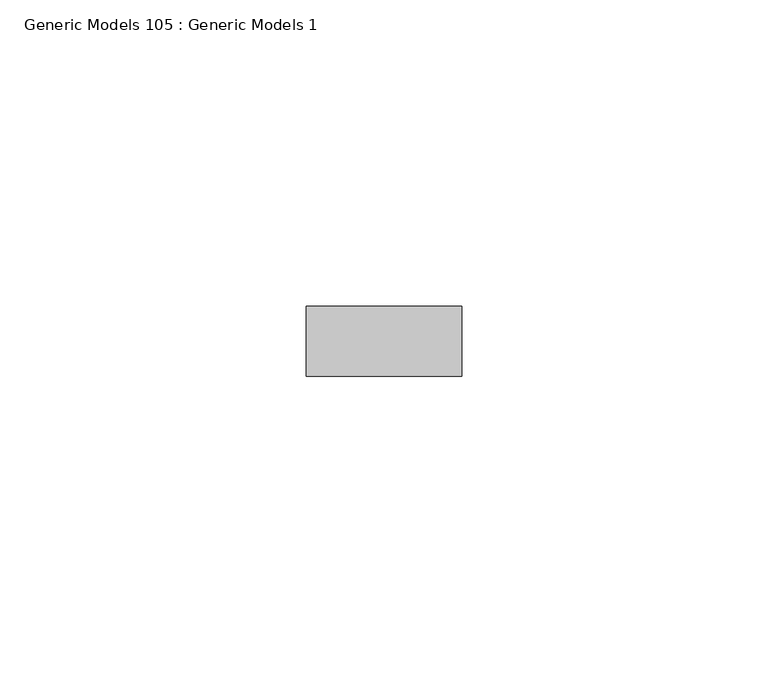
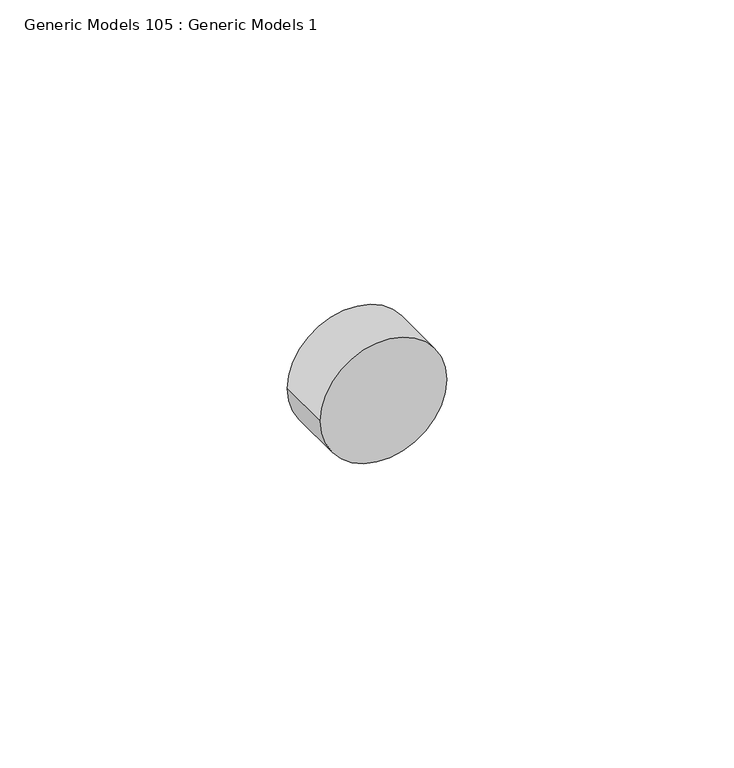
"""IFC4 building model written with IfcOpenShell, lengths in millimetres: proxy geometry, Generic Models 105 : Generic Models 1."""

import ifcopenshell
import ifcopenshell.guid

model = None  # the IFC model being written
_history = None  # IfcOwnerHistory: only IFC2X3 demands one
_inside = {}  # id of a spatial element -> (the spatial element, [elements in it])
_under = {}  # id of a project, library or spatial element -> (it, [spatial elements below it])
_declared = {}  # id of a project -> (the project, [libraries it declares])
_typed = {}  # id of a type object -> (the type object, [elements of that type])
_made_of = {}  # id of a material, layer set ... -> (it, [elements and type objects made of it])


def new_model(schema):
    """Start an empty IFC model of exactly this schema.

    Asked for "IFC4X3", IfcOpenShell would pick the latest addendum, in which some entities
    have other attributes; the version numbers below select the first issue.
    IFC2X3 requires an IfcOwnerHistory on every rooted entity: one is made here for all.
    """
    global model, _history
    if schema == "IFC4X3":
        model = ifcopenshell.file(schema_version=(4, 3, 0, 0))
    else:
        model = ifcopenshell.file(schema=schema)
    _inside.clear()
    _under.clear()
    _declared.clear()
    _typed.clear()
    _made_of.clear()
    _history = None
    if model.schema == "IFC2X3":
        org = make("IfcOrganization", Name="unknown")
        user = make(
            "IfcPersonAndOrganization",
            ThePerson=make("IfcPerson", FamilyName="unknown"),
            TheOrganization=org,
        )
        app = make(
            "IfcApplication",
            ApplicationDeveloper=org,
            Version="unknown",
            ApplicationFullName="unknown",
            ApplicationIdentifier="unknown",
        )
        _history = make(
            "IfcOwnerHistory",
            OwningUser=user,
            OwningApplication=app,
            ChangeAction="ADDED",
            CreationDate=0,
        )
    return model


def make(cls, **values):
    """One entity of the class cls with the attributes given. An attribute that is None is left unset."""
    return model.create_entity(
        cls, **{name: value for name, value in values.items() if value is not None}
    )


def rooted(cls, **values):
    """An entity with a GlobalId (a new one), such as an element, a storey or a relation."""
    return make(cls, GlobalId=ifcopenshell.guid.new(), OwnerHistory=_history, **values)


def si_unit(unit_type, name, prefix=None):
    """IfcSIUnit, for example si_unit("LENGTHUNIT", "METRE", prefix="MILLI")."""
    return make("IfcSIUnit", UnitType=unit_type, Prefix=prefix, Name=name)


def assignment(units):
    """IfcUnitAssignment: the units of a project."""
    return None if units is None else make("IfcUnitAssignment", Units=units)


def point(xyz):
    """IfcCartesianPoint."""
    return None if xyz is None else make("IfcCartesianPoint", Coordinates=xyz)


def direction(xyz):
    """IfcDirection."""
    return None if xyz is None else make("IfcDirection", DirectionRatios=xyz)


def frame(location, z_axis=None, x_axis=None):
    """IfcAxis2Placement3D, a coordinate frame: its origin and axes. An axis left out is left unset."""
    return make(
        "IfcAxis2Placement3D",
        Location=point(location),
        Axis=direction(z_axis),
        RefDirection=direction(x_axis),
    )


def frame_2d(location, x_axis=None):
    """IfcAxis2Placement2D, a coordinate frame in the plane: its origin and x axis."""
    return make(
        "IfcAxis2Placement2D", Location=point(location), RefDirection=direction(x_axis)
    )


def origin():
    """The frame at (0, 0, 0) with its axes left unset."""
    return frame((0.0, 0.0, 0.0))


def place(relative_to, where):
    """IfcLocalPlacement: puts the frame where relative to a parent placement (None: the world)."""
    return make(
        "IfcLocalPlacement", PlacementRelTo=relative_to, RelativePlacement=where
    )


def context(
    kind, dimensions, precision=None, world=None, true_north=None, identifier=None
):
    """IfcGeometricRepresentationContext, for example the 3D "Model" context."""
    return make(
        "IfcGeometricRepresentationContext",
        ContextIdentifier=identifier,
        ContextType=kind,
        CoordinateSpaceDimension=dimensions,
        Precision=precision,
        WorldCoordinateSystem=world,
        TrueNorth=true_north,
    )


def project(units=None, contexts=None):
    """IfcProject with its units and contexts."""
    return rooted(
        "IfcProject",
        Name="project",
        RepresentationContexts=contexts,
        UnitsInContext=assignment(units),
    )


def spatial(cls, under=None, at=None, **own):
    """A site, building, storey or space (cls), placed at a placement, below another one or the project."""
    s = rooted(cls, ObjectPlacement=at, **own)
    if under is not None:
        _under.setdefault(under.id(), (under, []))[1].append(s)
    return s


def circle_curve(where, radius):
    """IfcCircle in the frame where."""
    return make("IfcCircle", Position=where, Radius=radius)


def trimmed(basis, trim1, trim2, sense, master):
    """IfcTrimmedCurve: the piece of a basis curve between two trims."""
    return make(
        "IfcTrimmedCurve",
        BasisCurve=basis,
        Trim1=trim1,
        Trim2=trim2,
        SenseAgreement=sense,
        MasterRepresentation=master,
    )


def segment(curve, same_sense, transition):
    """IfcCompositeCurveSegment."""
    return make(
        "IfcCompositeCurveSegment",
        Transition=transition,
        SameSense=same_sense,
        ParentCurve=curve,
    )


def composite_curve(segments, self_intersect=None):
    """IfcCompositeCurve: segments joined end to end."""
    return make("IfcCompositeCurve", Segments=segments, SelfIntersect=self_intersect)


def outline(outer, holes=None, kind="AREA"):
    """IfcArbitraryClosedProfileDef: a profile drawn as a closed curve; with holes, ...WithVoids."""
    if holes is None:
        return make("IfcArbitraryClosedProfileDef", ProfileType=kind, OuterCurve=outer)
    return make(
        "IfcArbitraryProfileDefWithVoids",
        ProfileType=kind,
        OuterCurve=outer,
        InnerCurves=holes,
    )


def extrude(swept, where, along, depth):
    """IfcExtrudedAreaSolid: the profile swept, set in the frame where, extruded along a direction by depth."""
    return make(
        "IfcExtrudedAreaSolid",
        SweptArea=swept,
        Position=where,
        ExtrudedDirection=direction(along),
        Depth=depth,
    )


def shape(context_of_items, identifier, shape_type, items):
    """IfcShapeRepresentation: the items that make up one representation, for example the "Body"."""
    return make(
        "IfcShapeRepresentation",
        ContextOfItems=context_of_items,
        RepresentationIdentifier=identifier,
        RepresentationType=shape_type,
        Items=items,
    )


def source(mapping_origin, context_of_items, identifier, shape_type, items):
    """IfcRepresentationMap: a shape defined once, which mapped items show again and again."""
    return make(
        "IfcRepresentationMap",
        MappingOrigin=mapping_origin,
        MappedRepresentation=shape(context_of_items, identifier, shape_type, items),
    )


def transform(
    local_origin,
    x_axis=None,
    y_axis=None,
    z_axis=None,
    scale=None,
    scale2=None,
    scale3=None,
    uniform=True,
):
    """IfcCartesianTransformationOperator3D, or its non-uniform kind. x_axis, y_axis, z_axis: its Axis1, 2, 3."""
    if uniform:
        return make(
            "IfcCartesianTransformationOperator3D",
            Axis1=direction(x_axis),
            Axis2=direction(y_axis),
            LocalOrigin=point(local_origin),
            Scale=scale,
            Axis3=direction(z_axis),
        )
    return make(
        "IfcCartesianTransformationOperator3DnonUniform",
        Axis1=direction(x_axis),
        Axis2=direction(y_axis),
        LocalOrigin=point(local_origin),
        Scale=scale,
        Axis3=direction(z_axis),
        Scale2=scale2,
        Scale3=scale3,
    )


def mapped(mapping_source, mapping_target):
    """IfcMappedItem: shows the shape of a source again, moved by a transform."""
    return make(
        "IfcMappedItem", MappingSource=mapping_source, MappingTarget=mapping_target
    )


def made_of(thing, what):
    """Note that an element or type object is made of a material, layer set ...; save() writes the relation."""
    if what is not None:
        _made_of.setdefault(what.id(), (what, []))[1].append(thing)
    return thing


def element(
    cls,
    number,
    at=None,
    inside=None,
    cuts=None,
    type_object=None,
    material=None,
    context=None,
    identifier="Body",
    shape_type=None,
    held_by="IfcProductDefinitionShape",
    body=None,
    shapes=None,
    **own,
):
    """One element of the class cls, such as IfcWall. Its Tag is "e" and its number.

    at: its placement. inside: the storey or other place that contains it. cuts: it is an
    opening in that element (IfcRelVoidsElement). A single representation is given by context,
    identifier, shape_type and body (its items); several are given by shapes. held_by: the class
    of the entity that holds the representations. save() writes the other relations.
    """
    e = rooted(cls, Tag="e%d" % number, ObjectPlacement=at, **own)
    if body is not None:
        shapes = [shape(context, identifier, shape_type, body)]
    if shapes is not None:
        e.Representation = make(held_by, Representations=shapes)
    if inside is not None:
        _inside.setdefault(inside.id(), (inside, []))[1].append(e)
    if cuts is not None:
        rooted(
            "IfcRelVoidsElement", RelatingBuildingElement=cuts, RelatedOpeningElement=e
        )
    if type_object is not None:
        _typed.setdefault(type_object.id(), (type_object, []))[1].append(e)
    return made_of(e, material)


def aggregate(whole, parts):
    """IfcRelAggregates: a whole, such as a stair, and the parts it consists of."""
    return rooted("IfcRelAggregates", RelatingObject=whole, RelatedObjects=parts)


def save(model, path):
    """Write the relations noted so far, then the file.

    IfcRelAggregates (storeys below a building ...), IfcRelContainedInSpatialStructure (elements
    in a storey), IfcRelDefinesByType, IfcRelAssociatesMaterial and IfcRelDeclares: one each for
    every whole, place, type object, material and project.
    """
    for whole, parts in _under.values():
        aggregate(whole, parts)
    for where, things in _inside.values():
        rooted(
            "IfcRelContainedInSpatialStructure",
            RelatedElements=things,
            RelatingStructure=where,
        )
    for kind, things in _typed.values():
        rooted("IfcRelDefinesByType", RelatedObjects=things, RelatingType=kind)
    for what, things in _made_of.values():
        rooted("IfcRelAssociatesMaterial", RelatedObjects=things, RelatingMaterial=what)
    for by, libraries in _declared.values():
        rooted("IfcRelDeclares", RelatingContext=by, RelatedDefinitions=libraries)
    model.write(path)


def generic_models_105_generic_models_1_8c8b2fa9(model_context):
    return source(origin(), model_context, "Body", "SweptSolid", [
        extrude(outline(composite_curve([segment(trimmed(circle_curve(frame_2d((37517.3905034, 6289.9828124)), 12.7), [point((37517.3905034, 6277.2828124))], [point((37517.3905034, 6302.6828124))], False, "CARTESIAN"), True, "CONTINUOUS"), segment(trimmed(circle_curve(frame_2d((37517.3905034, 6289.9828124)), 12.7), [point((37517.3905034, 6302.6828124))], [point((37517.3905034, 6277.2828124))], False, "CARTESIAN"), True, "CONTINUOUS")], self_intersect=False)), frame((0.0, 1836.9202358, 0.0), z_axis=(0.0, 1.0, 0.0), x_axis=(0.0, 0.0, 1.0)), (0.0, 0.0, 1.0), 11.4464372),
    ])


if __name__ == "__main__":
    model = new_model("IFC4")
    model_context = context("Model", 3, world=origin())
    ifc_project = project(units=[si_unit("LENGTHUNIT", "METRE", prefix="MILLI")], contexts=[model_context])
    site = spatial("IfcSite", under=ifc_project)
    building = spatial("IfcBuilding", under=site)
    placement = place(None, origin())
    generic_models_105_generic_models_1_shape = generic_models_105_generic_models_1_8c8b2fa9(model_context)
    element("IfcBuildingElementProxy", 1, Name="Generic Models 105 : Generic Models 1", ObjectType="Generic Models 105 : Generic Models 1", at=placement, inside=building, context=model_context, shape_type="MappedRepresentation", body=[
        mapped(generic_models_105_generic_models_1_shape, transform((0.0, 0.0, 0.0), x_axis=(1.0, 0.0, 0.0), y_axis=(0.0, 1.0, 0.0), z_axis=(0.0, 0.0, 1.0))),
    ])
    save(model, "model.ifc")

# Revit data of these elements
# Element 1 (IfcBuildingElementProxy, "Generic Models 105 : Generic Models 1")
#   Materials on its faces: "S.S. LAG BOLT - SEE STRUCT. DWGS"
# Materials
#   "S.S. LAG BOLT - SEE STRUCT. DWGS": class "Generic", colour RGB 120 120 120, transparency 0, Cost = 0
